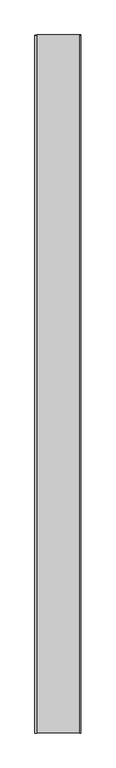
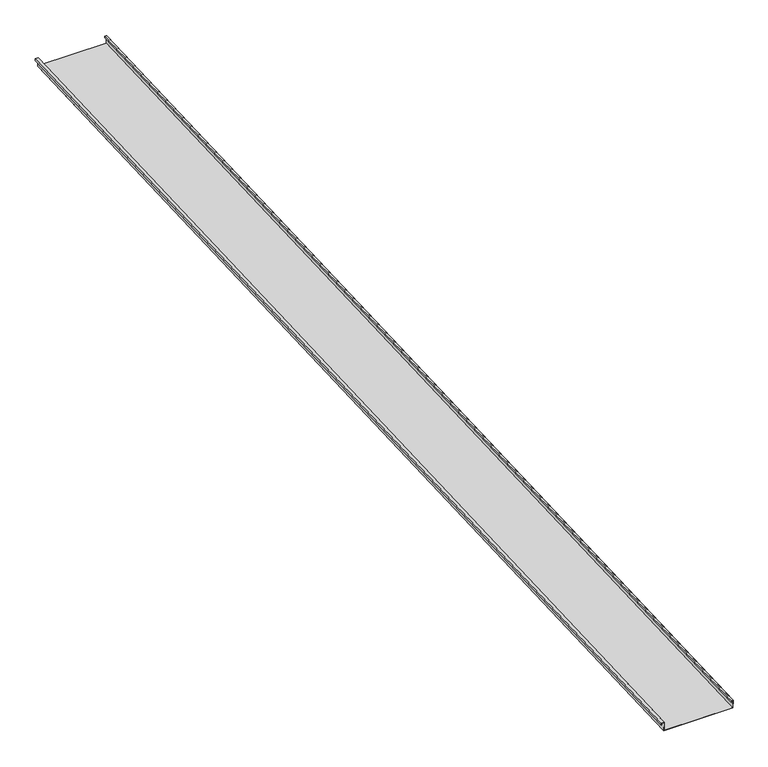
"""IFC4 building model written with IfcOpenShell, lengths in millimetres: proxy geometry, Generic Models 2:Generic Models 2:310765:Generic Models 2:310765 : Generic Models 2:Generic Models 2:310765:109 : Generic Models 2:Generic Models 2:310765:Generic Models 2:310765 : Generic Models 2:Generic Models 2:310765:300385."""

from ifc_helpers import new_model, si_unit, frame, origin, place, context, project, spatial, polyline, outline, extrude, source, transform, mapped, element, save


def generic_models_1d5e8461(model_context):
    return source(origin(), model_context, "Body", "SweptSolid", [
        extrude(outline(polyline([(1.5875, 0.0), (1.5875, 50.8), (407.9875, 50.8), (407.9875, 1.5875), (396.875, 1.5875), (396.875, 11.1125), (398.4625, 11.1125), (398.4625, 3.175), (406.4, 3.175), (406.4, 49.2125), (3.175, 49.2125), (3.175, -1.5874999), (-14.2875, -1.5874999), (-14.2875, 9.525), (-12.7, 9.525), (-12.7, 0.0), (1.5875, 0.0)])), frame((608651.3263073, -581354.4345603, 3902.6697972), z_axis=(0.0, 0.9991330730923568, 0.041630544712067834), x_axis=(1.0, 0.0, 0.0)), (0.0, 0.0, 1.0), 6400.8),
    ])


if __name__ == "__main__":
    model = new_model("IFC4")
    model_context = context("Model", 3, world=origin())
    ifc_project = project(units=[si_unit("LENGTHUNIT", "METRE", prefix="MILLI")], contexts=[model_context])
    site = spatial("IfcSite", under=ifc_project)
    building = spatial("IfcBuilding", under=site)
    placement = place(None, origin())
    generic_models_shape = generic_models_1d5e8461(model_context)
    element("IfcBuildingElementProxy", 1, Name="Generic Models 2:Generic Models 2:310765:Generic Models 2:310765 : Generic Models 2:Generic Models 2:310765:109 : Generic Models 2:Generic Models 2:310765:Generic Models 2:310765 : Generic Models 2:Generic Models 2:310765:300385", ObjectType="Generic Models 2:Generic Models 2:310765:Generic Models 2:310765 : Generic Models 2:Generic Models 2:310765:109 : Generic Models 2:Generic Models 2:310765:Generic Models 2:310765 : Generic Models 2:Generic Models 2:310765:300385", at=placement, inside=building, context=model_context, shape_type="MappedRepresentation", body=[
        mapped(generic_models_shape, transform((0.0, 0.0, 0.0), x_axis=(1.0, 0.0, 0.0), y_axis=(0.0, 1.0, 0.0), z_axis=(0.0, 0.0, 1.0))),
    ])
    save(model, "model.ifc")

# Revit data of these elements
# Type "Generic Models 2:Generic Models 2:310765:Generic Models 2:310765 : Generic Models 2:Generic Models 2:310765:109 : Generic Models 2:Generic Models 2:310765:Generic Models 2:310765 : Generic Models 2:Generic Models 2:310765:300385"
#   NameOverride = "Generic Models 2:Generic Models 2:310765:Generic Models 2:310765 : Generic Models 2:Generic Models 2:310765:300385"
#   ObjectTypeOverride = "Generic Models 2:310765 : Generic Models 2:Generic Models 2:310765"
#   Reference = "Generic Models 2"
#   Tag = "300385"
# Element 1 (IfcBuildingElementProxy, "Generic Models 2:Generic Models 2:310765:Generic Models 2:310765 : Generic Models 2:Generic Models 2:310765:109 : Generic Models 2:Generic Models 2:310765:Generic Models 2:310765 : Generic Models 2:Generic Models 2:310765:300385")
#   Materials on its faces: "THERMAL BROKEN ALUMINUM STOREFRONT FOR POLYCARBONATE"
# Materials
#   "THERMAL BROKEN ALUMINUM STOREFRONT FOR POLYCARBONATE": class "Unassigned", colour RGB 244 244 244, transparency 0, Keynote = "M07611300.01", Cost = 0
